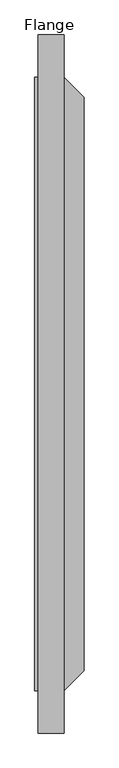
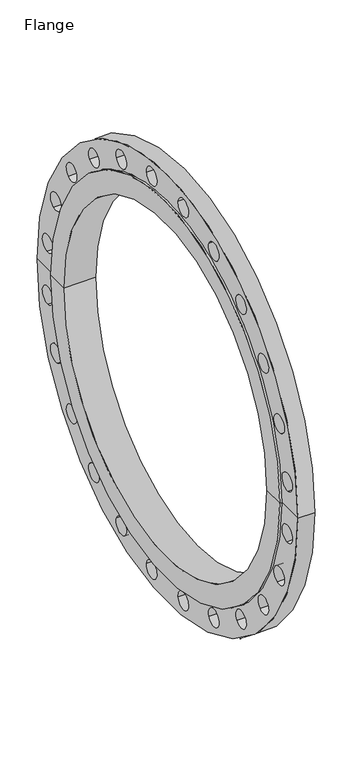
"""IFC4 building model written with IfcOpenShell, lengths in millimetres: proxy geometry, Flange : CASTED FLANGE PN16."""

from ifc_helpers import new_model, si_unit, frame, origin, place, context, project, spatial, polyline, circle_curve, source, transform, mapped, element, save
from ifc_brep_helpers import plane_surface, cylinder_surface, revolved_surface, advanced_brep


def flange_f2916e97(model_context):
    return source(origin(), model_context, "Body", "AdvancedBrep", [
        advanced_brep(
        [(0.0, 400.0, 0.0), (0.0, 450.5, 0.0), (0.0, -450.5, 0.0), (0.0, -400.0, 0.0), (72.5, 400.0, 0.0), (72.5, -400.0, 0.0), (72.5, 421.0, 0.0), (72.5, -421.0, 0.0), (43.0, 450.5, 0.0), (43.0, -450.5, 0.0), (43.0, 512.5, 0.0), (43.0, -512.5, 0.0), (43.0, -82.324561, -468.2605222), (43.0, -41.6753216, -473.6120961), (43.0, 41.6753216, -473.6120961), (43.0, 82.324561, -468.2605222), (43.0, -200.7141608, -430.9977676), (43.0, -162.8351, -446.6877883), (43.0, -305.4254223, -364.3632273), (43.0, -272.8979353, -389.3224459), (43.0, -389.3224459, -272.8979353), (43.0, -364.3632273, -305.4254223), (43.0, -446.6877883, -162.8351), (43.0, -430.9977676, -200.7141608), (43.0, -473.6120961, -41.6753216), (43.0, -468.2605222, -82.324561), (43.0, 468.2605222, -82.324561), (43.0, 473.6120961, -41.6753216), (43.0, 272.8979353, -389.3224459), (43.0, 305.4254223, -364.3632273), (43.0, 162.8351, -446.6877883), (43.0, 200.7141608, -430.9977676), (43.0, 430.9977676, -200.7141608), (43.0, 446.6877883, -162.8351), (43.0, 364.3632273, -305.4254223), (43.0, 389.3224459, -272.8979353), (43.0, -468.2605222, 82.324561), (43.0, -473.6120961, 41.6753216), (43.0, -272.8979353, 389.3224459), (43.0, -305.4254223, 364.3632273), (43.0, -162.8351, 446.6877883), (43.0, -200.7141608, 430.9977676), (43.0, -41.6753216, 473.6120961), (43.0, -82.324561, 468.2605222), (43.0, 82.324561, 468.2605222), (43.0, 41.6753216, 473.6120961), (43.0, 200.7141608, 430.9977676), (43.0, 162.8351, 446.6877883), (43.0, 305.4254223, 364.3632273), (43.0, 272.8979353, 389.3224459), (43.0, 389.3224459, 272.8979353), (43.0, 364.3632273, 305.4254223), (43.0, 446.6877883, 162.8351), (43.0, 430.9977676, 200.7141608), (43.0, 473.6120961, 41.6753216), (43.0, 468.2605222, 82.324561), (43.0, -430.9977676, 200.7141608), (43.0, -446.6877883, 162.8351), (43.0, -364.3632273, 305.4254223), (43.0, -389.3224459, 272.8979353), (5.0, 512.5, 0.0), (5.0, -512.5, 0.0), (5.0, 450.5, 0.0), (5.0, -450.5, 0.0), (5.0, -41.6753216, -473.6120961), (5.0, -82.324561, -468.2605222), (5.0, 82.324561, -468.2605222), (5.0, 41.6753216, -473.6120961), (5.0, -162.8351, -446.6877883), (5.0, -200.7141608, -430.9977676), (5.0, -272.8979353, -389.3224459), (5.0, -305.4254223, -364.3632273), (5.0, -364.3632273, -305.4254223), (5.0, -389.3224459, -272.8979353), (5.0, -430.9977676, -200.7141608), (5.0, -446.6877883, -162.8351), (5.0, -468.2605222, -82.324561), (5.0, -473.6120961, -41.6753216), (5.0, 473.6120961, -41.6753216), (5.0, 468.2605222, -82.324561), (5.0, 305.4254223, -364.3632273), (5.0, 272.8979353, -389.3224459), (5.0, 200.7141608, -430.9977676), (5.0, 162.8351, -446.6877883), (5.0, 446.6877883, -162.8351), (5.0, 430.9977676, -200.7141608), (5.0, 389.3224459, -272.8979353), (5.0, 364.3632273, -305.4254223), (5.0, -473.6120961, 41.6753216), (5.0, -468.2605222, 82.324561), (5.0, -305.4254223, 364.3632273), (5.0, -272.8979353, 389.3224459), (5.0, -200.7141608, 430.9977676), (5.0, -162.8351, 446.6877883), (5.0, -82.324561, 468.2605222), (5.0, -41.6753216, 473.6120961), (5.0, 41.6753216, 473.6120961), (5.0, 82.324561, 468.2605222), (5.0, 162.8351, 446.6877883), (5.0, 200.7141608, 430.9977676), (5.0, 272.8979353, 389.3224459), (5.0, 305.4254223, 364.3632273), (5.0, 364.3632273, 305.4254223), (5.0, 389.3224459, 272.8979353), (5.0, 430.9977676, 200.7141608), (5.0, 446.6877883, 162.8351), (5.0, 468.2605222, 82.324561), (5.0, 473.6120961, 41.6753216), (5.0, -446.6877883, 162.8351), (5.0, -430.9977676, 200.7141608), (5.0, -389.3224459, 272.8979353), (5.0, -364.3632273, 305.4254223)],
        [
            (0, 1),
            (1, 2, circle_curve(frame((0.0, 0.0, 0.0), z_axis=(-1.0, 0.0, 0.0), x_axis=(0.0, 1.0, 0.0)), 450.5)),
            (2, 3),
            (3, 0, circle_curve(frame((0.0, 0.0, 0.0), z_axis=(1.0, 0.0, 0.0), x_axis=(0.0, 1.0, 0.0)), 400.0)),
            (0, 3, circle_curve(frame((0.0, 0.0, 0.0), z_axis=(1.0, 0.0, 0.0), x_axis=(0.0, 1.0, 0.0)), 400.0)),
            (2, 1, circle_curve(frame((0.0, 0.0, 0.0), z_axis=(-1.0, 0.0, 0.0), x_axis=(0.0, 1.0, 0.0)), 450.5)),
            (4, 0),
            (3, 5),
            (5, 4, circle_curve(frame((72.5, 0.0, 0.0), z_axis=(1.0, 0.0, 0.0), x_axis=(0.0, 1.0, 0.0)), 400.0)),
            (4, 5, circle_curve(frame((72.5, 0.0, 0.0), z_axis=(1.0, 0.0, 0.0), x_axis=(0.0, 1.0, 0.0)), 400.0)),
            (6, 4),
            (5, 7),
            (7, 6, circle_curve(frame((72.5, 0.0, 0.0), z_axis=(1.0, 0.0, 0.0), x_axis=(0.0, 1.0, 0.0)), 421.0)),
            (6, 7, circle_curve(frame((72.5, 0.0, 0.0), z_axis=(1.0, 0.0, 0.0), x_axis=(0.0, 1.0, 0.0)), 421.0)),
            (8, 6),
            (7, 9),
            (9, 8, circle_curve(frame((43.0, 0.0, 0.0), z_axis=(1.0, 0.0, 0.0), x_axis=(0.0, 1.0, 0.0)), 450.5)),
            (8, 9, circle_curve(frame((43.0, 0.0, 0.0), z_axis=(1.0, 0.0, 0.0), x_axis=(0.0, 1.0, 0.0)), 450.5)),
            (10, 8),
            (9, 11),
            (11, 10, circle_curve(frame((43.0, 0.0, 0.0), z_axis=(1.0, 0.0, 0.0), x_axis=(0.0, 1.0, 0.0)), 512.5)),
            (12, 13, circle_curve(frame((43.0, -61.9999413, -470.9363092), z_axis=(-1.0, 0.0, 0.0), x_axis=(0.0, 0.9914448613738129, -0.13052619222003253)), 20.5)),
            (13, 12, circle_curve(frame((43.0, -61.9999413, -470.9363092), z_axis=(-1.0, 0.0, 0.0), x_axis=(0.0, 0.9914448613738129, -0.13052619222003253)), 20.5)),
            (14, 15, circle_curve(frame((43.0, 61.9999413, -470.9363092), z_axis=(-1.0, 0.0, 0.0), x_axis=(0.0, 0.9914448613738089, 0.13052619222006298)), 20.5)),
            (15, 14, circle_curve(frame((43.0, 61.9999413, -470.9363092), z_axis=(-1.0, 0.0, 0.0), x_axis=(0.0, 0.9914448613738089, 0.13052619222006298)), 20.5)),
            (16, 17, circle_curve(frame((43.0, -181.7746304, -438.8427779), z_axis=(-1.0, 0.0, 0.0), x_axis=(0.0, 0.9238795325113015, -0.38268343236505475)), 20.5)),
            (17, 16, circle_curve(frame((43.0, -181.7746304, -438.8427779), z_axis=(-1.0, 0.0, 0.0), x_axis=(0.0, 0.9238795325113015, -0.38268343236505475)), 20.5)),
            (18, 19, circle_curve(frame((43.0, -289.1616788, -376.8428366), z_axis=(-1.0, 0.0, 0.0), x_axis=(0.0, 0.7933533402912514, -0.6087614290086997)), 20.5)),
            (19, 18, circle_curve(frame((43.0, -289.1616788, -376.8428366), z_axis=(-1.0, 0.0, 0.0), x_axis=(0.0, 0.7933533402912514, -0.6087614290086997)), 20.5)),
            (20, 21, circle_curve(frame((43.0, -376.8428366, -289.1616788), z_axis=(-1.0, 0.0, 0.0), x_axis=(0.0, 0.6087614290087368, -0.793353340291223)), 20.5)),
            (21, 20, circle_curve(frame((43.0, -376.8428366, -289.1616788), z_axis=(-1.0, 0.0, 0.0), x_axis=(0.0, 0.6087614290087368, -0.793353340291223)), 20.5)),
            (22, 23, circle_curve(frame((43.0, -438.8427779, -181.7746304), z_axis=(-1.0, 0.0, 0.0), x_axis=(0.0, 0.3826834323651087, -0.923879532511279)), 20.5)),
            (23, 22, circle_curve(frame((43.0, -438.8427779, -181.7746304), z_axis=(-1.0, 0.0, 0.0), x_axis=(0.0, 0.3826834323651087, -0.923879532511279)), 20.5)),
            (24, 25, circle_curve(frame((43.0, -470.9363092, -61.9999413), z_axis=(-1.0, 0.0, 0.0), x_axis=(0.0, 0.130526192220072, -0.9914448613738078)), 20.5)),
            (25, 24, circle_curve(frame((43.0, -470.9363092, -61.9999413), z_axis=(-1.0, 0.0, 0.0), x_axis=(0.0, 0.130526192220072, -0.9914448613738078)), 20.5)),
            (26, 27, circle_curve(frame((43.0, 470.9363092, -61.9999413), z_axis=(-1.0, 0.0, 0.0), x_axis=(0.0, 0.13052619222001557, 0.9914448613738153)), 20.5)),
            (27, 26, circle_curve(frame((43.0, 470.9363092, -61.9999413), z_axis=(-1.0, 0.0, 0.0), x_axis=(0.0, 0.13052619222001557, 0.9914448613738153)), 20.5)),
            (28, 29, circle_curve(frame((43.0, 289.1616788, -376.8428366), z_axis=(-1.0, 0.0, 0.0), x_axis=(0.0, 0.7933533402912125, 0.6087614290087502)), 20.5)),
            (29, 28, circle_curve(frame((43.0, 289.1616788, -376.8428366), z_axis=(-1.0, 0.0, 0.0), x_axis=(0.0, 0.7933533402912125, 0.6087614290087502)), 20.5)),
            (30, 31, circle_curve(frame((43.0, 181.7746304, -438.8427779), z_axis=(-1.0, 0.0, 0.0), x_axis=(0.0, 0.9238795325112725, 0.3826834323651245)), 20.5)),
            (31, 30, circle_curve(frame((43.0, 181.7746304, -438.8427779), z_axis=(-1.0, 0.0, 0.0), x_axis=(0.0, 0.9238795325112725, 0.3826834323651245)), 20.5)),
            (32, 33, circle_curve(frame((43.0, 438.8427779, -181.7746304), z_axis=(-1.0, 0.0, 0.0), x_axis=(0.0, 0.38268343236505586, 0.9238795325113008)), 20.5)),
            (33, 32, circle_curve(frame((43.0, 438.8427779, -181.7746304), z_axis=(-1.0, 0.0, 0.0), x_axis=(0.0, 0.38268343236505586, 0.9238795325113008)), 20.5)),
            (34, 35, circle_curve(frame((43.0, 376.8428366, -289.1616788), z_axis=(-1.0, 0.0, 0.0), x_axis=(0.0, 0.6087614290086916, 0.7933533402912578)), 20.5)),
            (35, 34, circle_curve(frame((43.0, 376.8428366, -289.1616788), z_axis=(-1.0, 0.0, 0.0), x_axis=(0.0, 0.6087614290086916, 0.7933533402912578)), 20.5)),
            (10, 11, circle_curve(frame((43.0, 0.0, 0.0), z_axis=(1.0, 0.0, 0.0), x_axis=(0.0, 1.0, 0.0)), 512.5)),
            (36, 37, circle_curve(frame((43.0, -470.9363092, 61.9999413), z_axis=(-1.0, 0.0, 0.0), x_axis=(0.0, -0.13052619222003067, -0.9914448613738133)), 20.5)),
            (37, 36, circle_curve(frame((43.0, -470.9363092, 61.9999413), z_axis=(-1.0, 0.0, 0.0), x_axis=(0.0, -0.13052619222003067, -0.9914448613738133)), 20.5)),
            (38, 39, circle_curve(frame((43.0, -289.1616788, 376.8428366), z_axis=(-1.0, 0.0, 0.0), x_axis=(0.0, -0.7933533402912221, -0.6087614290087378)), 20.5)),
            (39, 38, circle_curve(frame((43.0, -289.1616788, 376.8428366), z_axis=(-1.0, 0.0, 0.0), x_axis=(0.0, -0.7933533402912221, -0.6087614290087378)), 20.5)),
            (40, 41, circle_curve(frame((43.0, -181.7746304, 438.8427779), z_axis=(-1.0, 0.0, 0.0), x_axis=(0.0, -0.9238795325112785, -0.38268343236510993)), 20.5)),
            (41, 40, circle_curve(frame((43.0, -181.7746304, 438.8427779), z_axis=(-1.0, 0.0, 0.0), x_axis=(0.0, -0.9238795325112785, -0.38268343236510993)), 20.5)),
            (42, 43, circle_curve(frame((43.0, -61.9999413, 470.9363092), z_axis=(-1.0, 0.0, 0.0), x_axis=(0.0, -0.9914448613738076, -0.1305261922200736)), 20.5)),
            (43, 42, circle_curve(frame((43.0, -61.9999413, 470.9363092), z_axis=(-1.0, 0.0, 0.0), x_axis=(0.0, -0.9914448613738076, -0.1305261922200736)), 20.5)),
            (44, 45, circle_curve(frame((43.0, 61.9999413, 470.9363092), z_axis=(-1.0, 0.0, 0.0), x_axis=(0.0, -0.9914448613738134, 0.13052619222002934)), 20.5)),
            (45, 44, circle_curve(frame((43.0, 61.9999413, 470.9363092), z_axis=(-1.0, 0.0, 0.0), x_axis=(0.0, -0.9914448613738134, 0.13052619222002934)), 20.5)),
            (46, 47, circle_curve(frame((43.0, 181.7746304, 438.8427779), z_axis=(-1.0, 0.0, 0.0), x_axis=(0.0, -0.9238795325113007, 0.3826834323650564)), 20.5)),
            (47, 46, circle_curve(frame((43.0, 181.7746304, 438.8427779), z_axis=(-1.0, 0.0, 0.0), x_axis=(0.0, -0.9238795325113007, 0.3826834323650564)), 20.5)),
            (48, 49, circle_curve(frame((43.0, 289.1616788, 376.8428366), z_axis=(-1.0, 0.0, 0.0), x_axis=(0.0, -0.7933533402912568, 0.6087614290086926)), 20.5)),
            (49, 48, circle_curve(frame((43.0, 289.1616788, 376.8428366), z_axis=(-1.0, 0.0, 0.0), x_axis=(0.0, -0.7933533402912568, 0.6087614290086926)), 20.5)),
            (50, 51, circle_curve(frame((43.0, 376.8428366, 289.1616788), z_axis=(-1.0, 0.0, 0.0), x_axis=(0.0, -0.6087614290087492, 0.7933533402912134)), 20.5)),
            (51, 50, circle_curve(frame((43.0, 376.8428366, 289.1616788), z_axis=(-1.0, 0.0, 0.0), x_axis=(0.0, -0.6087614290087492, 0.7933533402912134)), 20.5)),
            (52, 53, circle_curve(frame((43.0, 438.8427779, 181.7746304), z_axis=(-1.0, 0.0, 0.0), x_axis=(0.0, -0.38268343236512353, 0.923879532511273)), 20.5)),
            (53, 52, circle_curve(frame((43.0, 438.8427779, 181.7746304), z_axis=(-1.0, 0.0, 0.0), x_axis=(0.0, -0.38268343236512353, 0.923879532511273)), 20.5)),
            (54, 55, circle_curve(frame((43.0, 470.9363092, 61.9999413), z_axis=(-1.0, 0.0, 0.0), x_axis=(0.0, -0.13052619222008732, 0.9914448613738058)), 20.5)),
            (55, 54, circle_curve(frame((43.0, 470.9363092, 61.9999413), z_axis=(-1.0, 0.0, 0.0), x_axis=(0.0, -0.13052619222008732, 0.9914448613738058)), 20.5)),
            (56, 57, circle_curve(frame((43.0, -438.8427779, 181.7746304), z_axis=(-1.0, 0.0, 0.0), x_axis=(0.0, -0.3826834323650704, -0.9238795325112948)), 20.5)),
            (57, 56, circle_curve(frame((43.0, -438.8427779, 181.7746304), z_axis=(-1.0, 0.0, 0.0), x_axis=(0.0, -0.3826834323650704, -0.9238795325112948)), 20.5)),
            (58, 59, circle_curve(frame((43.0, -376.8428366, 289.1616788), z_axis=(-1.0, 0.0, 0.0), x_axis=(0.0, -0.6087614290087036, -0.7933533402912484)), 20.5)),
            (59, 58, circle_curve(frame((43.0, -376.8428366, 289.1616788), z_axis=(-1.0, 0.0, 0.0), x_axis=(0.0, -0.6087614290087036, -0.7933533402912484)), 20.5)),
            (60, 10),
            (11, 61),
            (61, 60, circle_curve(frame((5.0, 0.0, 0.0), z_axis=(1.0, 0.0, 0.0), x_axis=(0.0, 1.0, 0.0)), 512.5)),
            (60, 61, circle_curve(frame((5.0, 0.0, 0.0), z_axis=(1.0, 0.0, 0.0), x_axis=(0.0, 1.0, 0.0)), 512.5)),
            (62, 60),
            (61, 63),
            (63, 62, circle_curve(frame((5.0, 0.0, 0.0), z_axis=(1.0, 0.0, 0.0), x_axis=(0.0, 1.0, 0.0)), 450.5)),
            (64, 65, circle_curve(frame((5.0, -61.9999413, -470.9363092), z_axis=(1.0, 0.0, 0.0), x_axis=(0.0, 0.9914448613738129, -0.13052619222003253)), 20.5)),
            (65, 64, circle_curve(frame((5.0, -61.9999413, -470.9363092), z_axis=(1.0, 0.0, 0.0), x_axis=(0.0, 0.9914448613738129, -0.13052619222003253)), 20.5)),
            (66, 67, circle_curve(frame((5.0, 61.9999413, -470.9363092), z_axis=(1.0, 0.0, 0.0), x_axis=(0.0, 0.9914448613738089, 0.13052619222006298)), 20.5)),
            (67, 66, circle_curve(frame((5.0, 61.9999413, -470.9363092), z_axis=(1.0, 0.0, 0.0), x_axis=(0.0, 0.9914448613738089, 0.13052619222006298)), 20.5)),
            (68, 69, circle_curve(frame((5.0, -181.7746304, -438.8427779), z_axis=(1.0, 0.0, 0.0), x_axis=(0.0, 0.9238795325113015, -0.38268343236505475)), 20.5)),
            (69, 68, circle_curve(frame((5.0, -181.7746304, -438.8427779), z_axis=(1.0, 0.0, 0.0), x_axis=(0.0, 0.9238795325113015, -0.38268343236505475)), 20.5)),
            (70, 71, circle_curve(frame((5.0, -289.1616788, -376.8428366), z_axis=(1.0, 0.0, 0.0), x_axis=(0.0, 0.7933533402912514, -0.6087614290086997)), 20.5)),
            (71, 70, circle_curve(frame((5.0, -289.1616788, -376.8428366), z_axis=(1.0, 0.0, 0.0), x_axis=(0.0, 0.7933533402912514, -0.6087614290086997)), 20.5)),
            (72, 73, circle_curve(frame((5.0, -376.8428366, -289.1616788), z_axis=(1.0, 0.0, 0.0), x_axis=(0.0, 0.6087614290087368, -0.793353340291223)), 20.5)),
            (73, 72, circle_curve(frame((5.0, -376.8428366, -289.1616788), z_axis=(1.0, 0.0, 0.0), x_axis=(0.0, 0.6087614290087368, -0.793353340291223)), 20.5)),
            (74, 75, circle_curve(frame((5.0, -438.8427779, -181.7746304), z_axis=(1.0, 0.0, 0.0), x_axis=(0.0, 0.3826834323651087, -0.923879532511279)), 20.5)),
            (75, 74, circle_curve(frame((5.0, -438.8427779, -181.7746304), z_axis=(1.0, 0.0, 0.0), x_axis=(0.0, 0.3826834323651087, -0.923879532511279)), 20.5)),
            (76, 77, circle_curve(frame((5.0, -470.9363092, -61.9999413), z_axis=(1.0, 0.0, 0.0), x_axis=(0.0, 0.130526192220072, -0.9914448613738078)), 20.5)),
            (77, 76, circle_curve(frame((5.0, -470.9363092, -61.9999413), z_axis=(1.0, 0.0, 0.0), x_axis=(0.0, 0.130526192220072, -0.9914448613738078)), 20.5)),
            (78, 79, circle_curve(frame((5.0, 470.9363092, -61.9999413), z_axis=(1.0, 0.0, 0.0), x_axis=(0.0, 0.13052619222001557, 0.9914448613738153)), 20.5)),
            (79, 78, circle_curve(frame((5.0, 470.9363092, -61.9999413), z_axis=(1.0, 0.0, 0.0), x_axis=(0.0, 0.13052619222001557, 0.9914448613738153)), 20.5)),
            (80, 81, circle_curve(frame((5.0, 289.1616788, -376.8428366), z_axis=(1.0, 0.0, 0.0), x_axis=(0.0, 0.7933533402912125, 0.6087614290087502)), 20.5)),
            (81, 80, circle_curve(frame((5.0, 289.1616788, -376.8428366), z_axis=(1.0, 0.0, 0.0), x_axis=(0.0, 0.7933533402912125, 0.6087614290087502)), 20.5)),
            (82, 83, circle_curve(frame((5.0, 181.7746304, -438.8427779), z_axis=(1.0, 0.0, 0.0), x_axis=(0.0, 0.9238795325112725, 0.3826834323651245)), 20.5)),
            (83, 82, circle_curve(frame((5.0, 181.7746304, -438.8427779), z_axis=(1.0, 0.0, 0.0), x_axis=(0.0, 0.9238795325112725, 0.3826834323651245)), 20.5)),
            (84, 85, circle_curve(frame((5.0, 438.8427779, -181.7746304), z_axis=(1.0, 0.0, 0.0), x_axis=(0.0, 0.38268343236505586, 0.9238795325113008)), 20.5)),
            (85, 84, circle_curve(frame((5.0, 438.8427779, -181.7746304), z_axis=(1.0, 0.0, 0.0), x_axis=(0.0, 0.38268343236505586, 0.9238795325113008)), 20.5)),
            (86, 87, circle_curve(frame((5.0, 376.8428366, -289.1616788), z_axis=(1.0, 0.0, 0.0), x_axis=(0.0, 0.6087614290086916, 0.7933533402912578)), 20.5)),
            (87, 86, circle_curve(frame((5.0, 376.8428366, -289.1616788), z_axis=(1.0, 0.0, 0.0), x_axis=(0.0, 0.6087614290086916, 0.7933533402912578)), 20.5)),
            (62, 63, circle_curve(frame((5.0, 0.0, 0.0), z_axis=(1.0, 0.0, 0.0), x_axis=(0.0, 1.0, 0.0)), 450.5)),
            (88, 89, circle_curve(frame((5.0, -470.9363092, 61.9999413), z_axis=(1.0, 0.0, 0.0), x_axis=(0.0, -0.13052619222003067, -0.9914448613738133)), 20.5)),
            (89, 88, circle_curve(frame((5.0, -470.9363092, 61.9999413), z_axis=(1.0, 0.0, 0.0), x_axis=(0.0, -0.13052619222003067, -0.9914448613738133)), 20.5)),
            (90, 91, circle_curve(frame((5.0, -289.1616788, 376.8428366), z_axis=(1.0, 0.0, 0.0), x_axis=(0.0, -0.7933533402912221, -0.6087614290087378)), 20.5)),
            (91, 90, circle_curve(frame((5.0, -289.1616788, 376.8428366), z_axis=(1.0, 0.0, 0.0), x_axis=(0.0, -0.7933533402912221, -0.6087614290087378)), 20.5)),
            (92, 93, circle_curve(frame((5.0, -181.7746304, 438.8427779), z_axis=(1.0, 0.0, 0.0), x_axis=(0.0, -0.9238795325112785, -0.38268343236510993)), 20.5)),
            (93, 92, circle_curve(frame((5.0, -181.7746304, 438.8427779), z_axis=(1.0, 0.0, 0.0), x_axis=(0.0, -0.9238795325112785, -0.38268343236510993)), 20.5)),
            (94, 95, circle_curve(frame((5.0, -61.9999413, 470.9363092), z_axis=(1.0, 0.0, 0.0), x_axis=(0.0, -0.9914448613738076, -0.1305261922200736)), 20.5)),
            (95, 94, circle_curve(frame((5.0, -61.9999413, 470.9363092), z_axis=(1.0, 0.0, 0.0), x_axis=(0.0, -0.9914448613738076, -0.1305261922200736)), 20.5)),
            (96, 97, circle_curve(frame((5.0, 61.9999413, 470.9363092), z_axis=(1.0, 0.0, 0.0), x_axis=(0.0, -0.9914448613738134, 0.13052619222002934)), 20.5)),
            (97, 96, circle_curve(frame((5.0, 61.9999413, 470.9363092), z_axis=(1.0, 0.0, 0.0), x_axis=(0.0, -0.9914448613738134, 0.13052619222002934)), 20.5)),
            (98, 99, circle_curve(frame((5.0, 181.7746304, 438.8427779), z_axis=(1.0, 0.0, 0.0), x_axis=(0.0, -0.9238795325113007, 0.3826834323650564)), 20.5)),
            (99, 98, circle_curve(frame((5.0, 181.7746304, 438.8427779), z_axis=(1.0, 0.0, 0.0), x_axis=(0.0, -0.9238795325113007, 0.3826834323650564)), 20.5)),
            (100, 101, circle_curve(frame((5.0, 289.1616788, 376.8428366), z_axis=(1.0, 0.0, 0.0), x_axis=(0.0, -0.7933533402912568, 0.6087614290086926)), 20.5)),
            (101, 100, circle_curve(frame((5.0, 289.1616788, 376.8428366), z_axis=(1.0, 0.0, 0.0), x_axis=(0.0, -0.7933533402912568, 0.6087614290086926)), 20.5)),
            (102, 103, circle_curve(frame((5.0, 376.8428366, 289.1616788), z_axis=(1.0, 0.0, 0.0), x_axis=(0.0, -0.6087614290087492, 0.7933533402912134)), 20.5)),
            (103, 102, circle_curve(frame((5.0, 376.8428366, 289.1616788), z_axis=(1.0, 0.0, 0.0), x_axis=(0.0, -0.6087614290087492, 0.7933533402912134)), 20.5)),
            (104, 105, circle_curve(frame((5.0, 438.8427779, 181.7746304), z_axis=(1.0, 0.0, 0.0), x_axis=(0.0, -0.38268343236512353, 0.923879532511273)), 20.5)),
            (105, 104, circle_curve(frame((5.0, 438.8427779, 181.7746304), z_axis=(1.0, 0.0, 0.0), x_axis=(0.0, -0.38268343236512353, 0.923879532511273)), 20.5)),
            (106, 107, circle_curve(frame((5.0, 470.9363092, 61.9999413), z_axis=(1.0, 0.0, 0.0), x_axis=(0.0, -0.13052619222008732, 0.9914448613738058)), 20.5)),
            (107, 106, circle_curve(frame((5.0, 470.9363092, 61.9999413), z_axis=(1.0, 0.0, 0.0), x_axis=(0.0, -0.13052619222008732, 0.9914448613738058)), 20.5)),
            (108, 109, circle_curve(frame((5.0, -438.8427779, 181.7746304), z_axis=(1.0, 0.0, 0.0), x_axis=(0.0, -0.3826834323650704, -0.9238795325112948)), 20.5)),
            (109, 108, circle_curve(frame((5.0, -438.8427779, 181.7746304), z_axis=(1.0, 0.0, 0.0), x_axis=(0.0, -0.3826834323650704, -0.9238795325112948)), 20.5)),
            (110, 111, circle_curve(frame((5.0, -376.8428366, 289.1616788), z_axis=(1.0, 0.0, 0.0), x_axis=(0.0, -0.6087614290087036, -0.7933533402912484)), 20.5)),
            (111, 110, circle_curve(frame((5.0, -376.8428366, 289.1616788), z_axis=(1.0, 0.0, 0.0), x_axis=(0.0, -0.6087614290087036, -0.7933533402912484)), 20.5)),
            (1, 62),
            (63, 2),
            (12, 65),
            (64, 13),
            (14, 67),
            (66, 15),
            (16, 69),
            (68, 17),
            (18, 71),
            (70, 19),
            (20, 73),
            (72, 21),
            (22, 75),
            (74, 23),
            (24, 77),
            (76, 25),
            (36, 89),
            (88, 37),
            (56, 109),
            (108, 57),
            (58, 111),
            (110, 59),
            (38, 91),
            (90, 39),
            (40, 93),
            (92, 41),
            (42, 95),
            (94, 43),
            (44, 97),
            (96, 45),
            (46, 99),
            (98, 47),
            (48, 101),
            (100, 49),
            (50, 103),
            (102, 51),
            (52, 105),
            (104, 53),
            (54, 107),
            (106, 55),
            (26, 79),
            (78, 27),
            (32, 85),
            (84, 33),
            (34, 87),
            (86, 35),
            (28, 81),
            (80, 29),
            (30, 83),
            (82, 31),
        ],
        [
            plane_surface(frame((0.0, 0.0, 0.0), z_axis=(-1.0, 0.0, 0.0), x_axis=(0.0, 1.0, 0.0))),
            revolved_surface(polyline([(0.0, 400.0, 0.0), (72.5, 400.0, 0.0)]), (-95.0, 0.0, 0.0), (-1.0, 0.0, 0.0)),
            plane_surface(frame((72.5, 0.0, 0.0), z_axis=(1.0, 0.0, 0.0), x_axis=(0.0, 1.0, 0.0))),
            revolved_surface(polyline([(72.5, 421.0, 0.0), (43.0, 450.5, 0.0)]), (-95.0, 0.0, 0.0), (-1.0, 0.0, 0.0)),
            plane_surface(frame((43.0, 0.0, 0.0), z_axis=(1.0, 0.0, 0.0), x_axis=(0.0, 1.0, 0.0))),
            cylinder_surface(frame((-95.0, 0.0, 0.0), z_axis=(-1.0, 0.0, 0.0), x_axis=(0.0, 1.0, 0.0)), 512.5),
            plane_surface(frame((5.0, 0.0, 0.0), z_axis=(-1.0, 0.0, 0.0), x_axis=(0.0, 1.0, 0.0))),
            cylinder_surface(frame((-95.0, 0.0, 0.0), z_axis=(-1.0, 0.0, 0.0), x_axis=(0.0, 1.0, 0.0)), 450.5),
            revolved_surface(polyline([(5.0, -41.67532164183684, -473.61209614051063), (43.0, -41.67532164183684, -473.61209614051063)]), (43.0, -61.9999413, -470.9363092), (-1.0, 0.0, 0.0)),
            revolved_surface(polyline([(5.0, 82.32456095816309, -468.2605222594887), (43.0, 82.32456095816309, -468.2605222594887)]), (43.0, 61.9999413, -470.9363092), (-1.0, 0.0, 0.0)),
            revolved_surface(polyline([(4.999999999999986, -162.83509998351832, -446.6877882634836), (43.0, -162.83509998351832, -446.6877882634836)]), (43.0, -181.7746304, -438.8427779), (-1.0000000000000002, 0.0, 0.0)),
            revolved_surface(polyline([(5.0, -272.89793532402933, -389.32244589467837), (43.0, -272.89793532402933, -389.32244589467837)]), (43.0, -289.1616788, -376.8428366), (-1.0, 0.0, 0.0)),
            revolved_surface(polyline([(4.999999999999986, -364.3632273053209, -305.42542227597005), (43.0, -364.3632273053209, -305.42542227597005)]), (43.0, -376.8428366, -289.1616788), (-1.0000000000000002, 0.0, 0.0)),
            revolved_surface(polyline([(5.0, -430.99776753651525, -200.71416081648124), (43.0, -430.99776753651525, -200.71416081648124)]), (43.0, -438.8427779, -181.7746304), (-1.0, 0.0, 0.0)),
            revolved_surface(polyline([(5.0, -468.2605222594885, -82.32456095816306), (43.0, -468.2605222594885, -82.32456095816306)]), (43.0, -470.9363092, -61.9999413), (-1.0, 0.0, 0.0)),
            revolved_surface(polyline([(5.0, -473.61209614051063, 41.67532164183683), (43.0, -473.61209614051063, 41.67532164183683)]), (43.0, -470.9363092, 61.9999413), (-1.0, 0.0, 0.0)),
            revolved_surface(polyline([(5.0, -446.6877882634839, 162.83509998351846), (43.0, -446.6877882634839, 162.83509998351846)]), (43.0, -438.8427779, 181.7746304), (-1.0, 0.0, 0.0)),
            revolved_surface(polyline([(5.0, -389.3224458946784, 272.8979353240294), (43.0, -389.3224458946784, 272.8979353240294)]), (43.0, -376.8428366, 289.1616788), (-1.0, 0.0, 0.0)),
            revolved_surface(polyline([(5.0, -305.42542227597005, 364.3632273053209), (43.0, -305.42542227597005, 364.3632273053209)]), (43.0, -289.1616788, 376.8428366), (-1.0, 0.0, 0.0)),
            revolved_surface(polyline([(5.0, -200.7141608164812, 430.99776753651525), (43.0, -200.7141608164812, 430.99776753651525)]), (43.0, -181.7746304, 438.8427779), (-1.0, 0.0, 0.0)),
            revolved_surface(polyline([(4.999999999999986, -82.32456095816306, 468.2605222594885), (43.0, -82.32456095816306, 468.2605222594885)]), (43.0, -61.9999413, 470.9363092), (-1.0000000000000002, 0.0, 0.0)),
            revolved_surface(polyline([(5.0, 41.67532164183683, 473.6120961405106), (43.0, 41.67532164183683, 473.6120961405106)]), (43.0, 61.9999413, 470.9363092), (-1.0, 0.0, 0.0)),
            revolved_surface(polyline([(5.0, 162.83509998351835, 446.68778826348364), (43.0, 162.83509998351835, 446.68778826348364)]), (43.0, 181.7746304, 438.8427779), (-1.0, 0.0, 0.0)),
            revolved_surface(polyline([(5.0, 272.8979353240292, 389.3224458946782), (43.0, 272.8979353240292, 389.3224458946782)]), (43.0, 289.1616788, 376.8428366), (-1.0, 0.0, 0.0)),
            revolved_surface(polyline([(5.0, 364.36322730532066, 305.4254222759699), (43.0, 364.36322730532066, 305.4254222759699)]), (43.0, 376.8428366, 289.1616788), (-1.0, 0.0, 0.0)),
            revolved_surface(polyline([(5.0, 430.99776753651497, 200.7141608164811), (43.0, 430.99776753651497, 200.7141608164811)]), (43.0, 438.8427779, 181.7746304), (-1.0, 0.0, 0.0)),
            revolved_surface(polyline([(4.999999999999986, 468.2605222594882, 82.32456095816302), (43.0, 468.2605222594882, 82.32456095816302)]), (43.0, 470.9363092, 61.9999413), (-1.0000000000000002, 0.0, 0.0)),
            revolved_surface(polyline([(5.0, 473.6120961405103, -41.67532164183679), (43.0, 473.6120961405103, -41.67532164183679)]), (43.0, 470.9363092, -61.9999413), (-1.0, 0.0, 0.0)),
            revolved_surface(polyline([(5.0, 446.68778826348364, -162.83509998351835), (43.0, 446.68778826348364, -162.83509998351835)]), (43.0, 438.8427779, -181.7746304), (-1.0, 0.0, 0.0)),
            revolved_surface(polyline([(4.999999999999986, 389.3224458946782, -272.8979353240292), (43.0, 389.3224458946782, -272.8979353240292)]), (43.0, 376.8428366, -289.1616788), (-1.0000000000000002, 0.0, 0.0)),
            revolved_surface(polyline([(5.0, 305.4254222759699, -364.3632273053206), (43.0, 305.4254222759699, -364.3632273053206)]), (43.0, 289.1616788, -376.8428366), (-1.0, 0.0, 0.0)),
            revolved_surface(polyline([(5.0, 200.7141608164811, -430.9977675365149), (43.0, 200.7141608164811, -430.9977675365149)]), (43.0, 181.7746304, -438.8427779), (-1.0, 0.0, 0.0)),
        ],
        [
            (0, [[1, 2, 3, 4]]),
            (0, [[-1, 5, -3, 6]]),
            (1, [[7, -4, 8, 9]]),
            (1, [[-7, 10, -8, -5]]),
            (2, [[11, -9, 12, 13]]),
            (2, [[-11, 14, -12, -10]]),
            (3, [[15, -13, 16, 17]]),
            (3, [[-15, 18, -16, -14]]),
            (4, [[19, -17, 20, 21], [22, 23], [24, 25], [26, 27], [28, 29], [30, 31], [32, 33], [34, 35], [36, 37], [38, 39], [40, 41], [42, 43], [44, 45]]),
            (4, [[-19, 46, -20, -18], [47, 48], [49, 50], [51, 52], [53, 54], [55, 56], [57, 58], [59, 60], [61, 62], [63, 64], [65, 66], [67, 68], [69, 70]]),
            (5, [[71, -21, 72, 73]]),
            (5, [[-71, 74, -72, -46]]),
            (6, [[75, -73, 76, 77], [78, 79], [80, 81], [82, 83], [84, 85], [86, 87], [88, 89], [90, 91], [92, 93], [94, 95], [96, 97], [98, 99], [100, 101]]),
            (6, [[-75, 102, -76, -74], [103, 104], [105, 106], [107, 108], [109, 110], [111, 112], [113, 114], [115, 116], [117, 118], [119, 120], [121, 122], [123, 124], [125, 126]]),
            (7, [[127, -77, 128, -2]]),
            (7, [[-127, -6, -128, -102]]),
            (8, [[129, -78, 130, -22]]),
            (8, [[-129, -23, -130, -79]]),
            (9, [[131, -80, 132, -24]]),
            (9, [[-131, -25, -132, -81]]),
            (10, [[133, -82, 134, -26]]),
            (10, [[-133, -27, -134, -83]]),
            (11, [[135, -84, 136, -28]]),
            (11, [[-135, -29, -136, -85]]),
            (12, [[137, -86, 138, -30]]),
            (12, [[-137, -31, -138, -87]]),
            (13, [[139, -88, 140, -32]]),
            (13, [[-139, -33, -140, -89]]),
            (14, [[141, -90, 142, -34]]),
            (14, [[-141, -35, -142, -91]]),
            (15, [[143, -103, 144, -47]]),
            (15, [[-143, -48, -144, -104]]),
            (16, [[145, -123, 146, -67]]),
            (16, [[-145, -68, -146, -124]]),
            (17, [[147, -125, 148, -69]]),
            (17, [[-147, -70, -148, -126]]),
            (18, [[149, -105, 150, -49]]),
            (18, [[-149, -50, -150, -106]]),
            (19, [[151, -107, 152, -51]]),
            (19, [[-151, -52, -152, -108]]),
            (20, [[153, -109, 154, -53]]),
            (20, [[-153, -54, -154, -110]]),
            (21, [[155, -111, 156, -55]]),
            (21, [[-155, -56, -156, -112]]),
            (22, [[157, -113, 158, -57]]),
            (22, [[-157, -58, -158, -114]]),
            (23, [[159, -115, 160, -59]]),
            (23, [[-159, -60, -160, -116]]),
            (24, [[161, -117, 162, -61]]),
            (24, [[-161, -62, -162, -118]]),
            (25, [[163, -119, 164, -63]]),
            (25, [[-163, -64, -164, -120]]),
            (26, [[165, -121, 166, -65]]),
            (26, [[-165, -66, -166, -122]]),
            (27, [[167, -92, 168, -36]]),
            (27, [[-167, -37, -168, -93]]),
            (28, [[169, -98, 170, -42]]),
            (28, [[-169, -43, -170, -99]]),
            (29, [[171, -100, 172, -44]]),
            (29, [[-171, -45, -172, -101]]),
            (30, [[173, -94, 174, -38]]),
            (30, [[-173, -39, -174, -95]]),
            (31, [[175, -96, 176, -40]]),
            (31, [[-175, -41, -176, -97]]),
        ],
    ),
    ])


if __name__ == "__main__":
    model = new_model("IFC4")
    model_context = context("Model", 3, world=origin())
    ifc_project = project(units=[si_unit("LENGTHUNIT", "METRE", prefix="MILLI")], contexts=[model_context])
    site = spatial("IfcSite", under=ifc_project)
    building = spatial("IfcBuilding", under=site)
    placement = place(None, origin())
    flange_shape = flange_f2916e97(model_context)
    element("IfcBuildingElementProxy", 1, Name="Flange : CASTED FLANGE PN16", ObjectType="Flange : CASTED FLANGE PN16", at=placement, inside=building, context=model_context, shape_type="MappedRepresentation", body=[
        mapped(flange_shape, transform((0.0, 0.0, 0.0), x_axis=(1.0, 0.0, 0.0), y_axis=(0.0, 1.0, 0.0), z_axis=(0.0, 0.0, 1.0))),
    ])
    save(model, "model.ifc")

# Revit data of these elements
# Project information
#   Company Address = "Fabriksvej 8, V. Lyby DK-7800 Skive"
#   Company E-mail = "info@aconsult.dk"
#   Company Phone = "+45 9687 5800"
#   Company Website = "www.aconsult.dk"
#   Concrete Strength = "CXX/XX"
#   Exposure Class = "XX"
#   Recept = "XX"
#   Kontrolklasse DK = "XX"
#   Panel Supplier = "Example - RC Beton"
#   Company Fax = "+45 9687 5858"
#   Organization Name = "A-CONSULT AGRO A/S"
#   Project Issue Date = "Issue Date"
#   Project Status = "FOR APPROVAL"
#   Client Name = "Client Name"
#   Project Address = "Enter address here"
#   Project Name = "Project Name"
#   Project Number = "XXXXXX"
# Type "Flange : CASTED FLANGE PN16"
#   TABLE_DIMENSIONS = "DIMENSIONS FIXED FLANGE"
#   Short Description = ""
#   Description = "FIXED FLANGE"
#   K [instance default] = 110 mm
#   HOLE DIAMETER [instance default] = 19 mm
#   D4 [instance default] = 84 mm
#   DRILL DIAMETER [instance default] = 110 mm
#   DN [instance default] = 40 mm
#   D2 [instance default] = 70 mm
#   D [instance default] = 150 mm
#   f [instance default] = 3 mm
#   b [instance default] = 16 mm
#   ANGLE [instance default] = 45.00°
#   a [instance default] = 19 mm
#   PN = 16
#   BOLTS NUMBER [instance default] = 4
#   MATERIAL [instance default] = none
#   COATING [instance default] = none
#   Default Elevation = 0
# Element 1 (IfcBuildingElementProxy, "Flange : CASTED FLANGE PN16")
#   K = 950 mm
#   HOLE DIAMETER = 41 mm
#   D4 = 901 mm
#   DRILL DIAMETER = 950 mm
#   DN = 800 mm
#   D2 = 842 mm
#   D = 1025 mm
#   f = 5 mm
#   b = 38 mm
#   a = 43 mm
#   BOLTS NUMBER = 24
#   COATING = Not informed
#   Materials on its faces: "Not informed"
# Materials
#   "Not informed": class "Paint/Coating", colour RGB 0 56 123, transparency 0, Description = "Not Informed", Cost = 0
